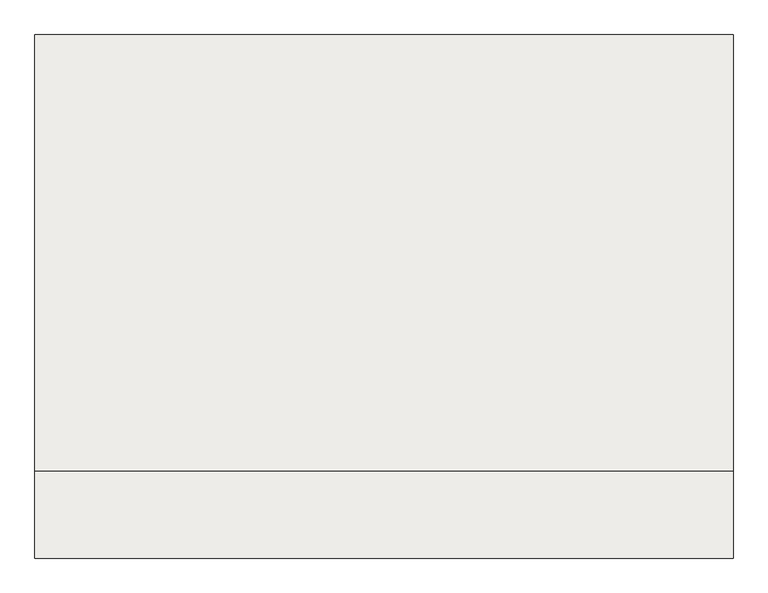
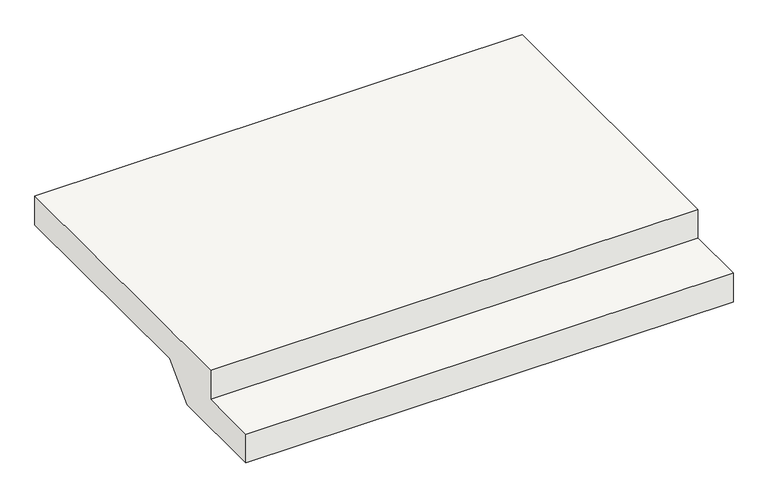
"""IFC4 building model written with IfcOpenShell, lengths in millimetres: slab geometry, Stoop : FTS901_STOOP."""

from ifc_helpers import new_model, si_unit, frame, origin, place, context, project, spatial, polyline, outline, extrude, source, transform, mapped, element, save


def slab_d684a698(model_context):
    return source(origin(), model_context, "Body", "SweptSolid", [
        extrude(outline(polyline([(-1800.0, 150.0), (-1500.0, 150.0), (-1500.0, 300.0), (0.0, 300.0), (0.0, 150.0), (-1150.0, 150.0), (-1300.0, 0.0), (-1800.0, 0.0), (-1800.0, 150.0)])), frame((-1200.0, 0.0, 0.0), z_axis=(1.0, 0.0, 0.0), x_axis=(0.0, 1.0, 0.0)), (0.0, 0.0, 1.0), 2400.0),
    ])


if __name__ == "__main__":
    model = new_model("IFC4")
    model_context = context("Model", 3, world=origin())
    ifc_project = project(units=[si_unit("LENGTHUNIT", "METRE", prefix="MILLI")], contexts=[model_context])
    site = spatial("IfcSite", under=ifc_project)
    building = spatial("IfcBuilding", under=site)
    placement = place(None, origin())
    slab_shape = slab_d684a698(model_context)
    element("IfcSlab", 1, ObjectType="Stoop : FTS901_STOOP", at=placement, inside=building, context=model_context, shape_type="MappedRepresentation", body=[
        mapped(slab_shape, transform((0.0, 0.0, 0.0), x_axis=(1.0, 0.0, 0.0), y_axis=(0.0, 1.0, 0.0), z_axis=(0.0, 0.0, 1.0))),
    ])
    save(model, "model.ifc")

# Revit data of these elements
# Type "Stoop : FTS901_STOOP"
#   Width = 2400 mm
#   Length = 1500 mm
#   Thickness = 150 mm
#   Structural Material = A03AC032-00007_Structural Concrete_Type1_25MPa-30Mpa
#   Default Elevation = 0
# Element 1 (IfcSlab, "Stoop : FTS901_STOOP")
#   Materials on its faces: "A03AC032-00007_Structural Concrete_Type1_25MPa-30Mpa"
# Materials
#   "A03AC032-00007_Structural Concrete_Type1_25MPa-30Mpa": class "Concrete", colour RGB 176 176 176, transparency 0, Keynote = "09910.A1", Description = "Reinf. Conc.", W00) Work Master Code = "A03AC032-00007", W01) Work Master_Lv1 = "Concrete Work", W02) Work Master_Lv2 = "Substructure Work", W03) Work Master_Spec.1 = "Structural Concrete", W04) Work Master_Spec.2 = "Cement Type-1", W05) Work Master_Spec.3 = "25MPa < F'c (Cylinder Strength) ≤ 30MPa", Cost = 0
